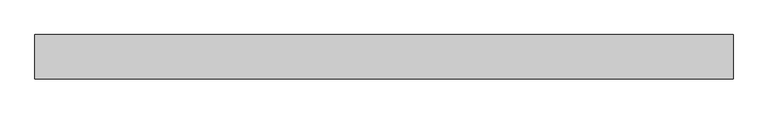
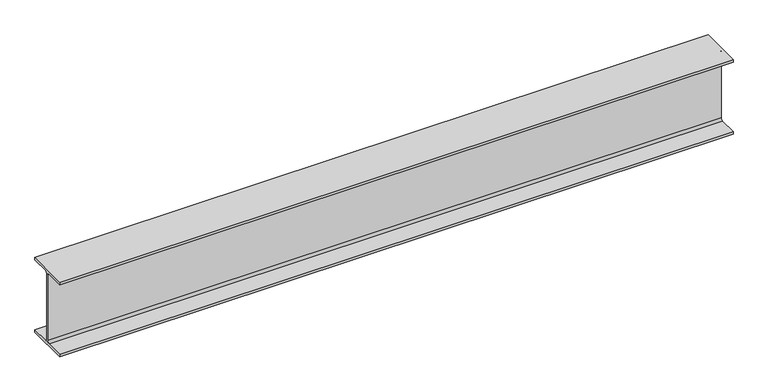
"""IFC4 building model written with IfcOpenShell, lengths in millimetres: beam geometry, Old_Steel Beam_H-KSD3502 : H_SB_ASB_H-250×125x6x9."""

import ifcopenshell
import ifcopenshell.guid

model = None  # the IFC model being written
_history = None  # IfcOwnerHistory: only IFC2X3 demands one
_inside = {}  # id of a spatial element -> (the spatial element, [elements in it])
_under = {}  # id of a project, library or spatial element -> (it, [spatial elements below it])
_declared = {}  # id of a project -> (the project, [libraries it declares])
_typed = {}  # id of a type object -> (the type object, [elements of that type])
_made_of = {}  # id of a material, layer set ... -> (it, [elements and type objects made of it])


def new_model(schema):
    """Start an empty IFC model of exactly this schema.

    Asked for "IFC4X3", IfcOpenShell would pick the latest addendum, in which some entities
    have other attributes; the version numbers below select the first issue.
    IFC2X3 requires an IfcOwnerHistory on every rooted entity: one is made here for all.
    """
    global model, _history
    if schema == "IFC4X3":
        model = ifcopenshell.file(schema_version=(4, 3, 0, 0))
    else:
        model = ifcopenshell.file(schema=schema)
    _inside.clear()
    _under.clear()
    _declared.clear()
    _typed.clear()
    _made_of.clear()
    _history = None
    if model.schema == "IFC2X3":
        org = make("IfcOrganization", Name="unknown")
        user = make(
            "IfcPersonAndOrganization",
            ThePerson=make("IfcPerson", FamilyName="unknown"),
            TheOrganization=org,
        )
        app = make(
            "IfcApplication",
            ApplicationDeveloper=org,
            Version="unknown",
            ApplicationFullName="unknown",
            ApplicationIdentifier="unknown",
        )
        _history = make(
            "IfcOwnerHistory",
            OwningUser=user,
            OwningApplication=app,
            ChangeAction="ADDED",
            CreationDate=0,
        )
    return model


def make(cls, **values):
    """One entity of the class cls with the attributes given. An attribute that is None is left unset."""
    return model.create_entity(
        cls, **{name: value for name, value in values.items() if value is not None}
    )


def rooted(cls, **values):
    """An entity with a GlobalId (a new one), such as an element, a storey or a relation."""
    return make(cls, GlobalId=ifcopenshell.guid.new(), OwnerHistory=_history, **values)


def si_unit(unit_type, name, prefix=None):
    """IfcSIUnit, for example si_unit("LENGTHUNIT", "METRE", prefix="MILLI")."""
    return make("IfcSIUnit", UnitType=unit_type, Prefix=prefix, Name=name)


def assignment(units):
    """IfcUnitAssignment: the units of a project."""
    return None if units is None else make("IfcUnitAssignment", Units=units)


def point(xyz):
    """IfcCartesianPoint."""
    return None if xyz is None else make("IfcCartesianPoint", Coordinates=xyz)


def direction(xyz):
    """IfcDirection."""
    return None if xyz is None else make("IfcDirection", DirectionRatios=xyz)


def frame(location, z_axis=None, x_axis=None):
    """IfcAxis2Placement3D, a coordinate frame: its origin and axes. An axis left out is left unset."""
    return make(
        "IfcAxis2Placement3D",
        Location=point(location),
        Axis=direction(z_axis),
        RefDirection=direction(x_axis),
    )


def frame_2d(location, x_axis=None):
    """IfcAxis2Placement2D, a coordinate frame in the plane: its origin and x axis."""
    return make(
        "IfcAxis2Placement2D", Location=point(location), RefDirection=direction(x_axis)
    )


def origin():
    """The frame at (0, 0, 0) with its axes left unset."""
    return frame((0.0, 0.0, 0.0))


def place(relative_to, where):
    """IfcLocalPlacement: puts the frame where relative to a parent placement (None: the world)."""
    return make(
        "IfcLocalPlacement", PlacementRelTo=relative_to, RelativePlacement=where
    )


def context(
    kind, dimensions, precision=None, world=None, true_north=None, identifier=None
):
    """IfcGeometricRepresentationContext, for example the 3D "Model" context."""
    return make(
        "IfcGeometricRepresentationContext",
        ContextIdentifier=identifier,
        ContextType=kind,
        CoordinateSpaceDimension=dimensions,
        Precision=precision,
        WorldCoordinateSystem=world,
        TrueNorth=true_north,
    )


def project(units=None, contexts=None):
    """IfcProject with its units and contexts."""
    return rooted(
        "IfcProject",
        Name="project",
        RepresentationContexts=contexts,
        UnitsInContext=assignment(units),
    )


def spatial(cls, under=None, at=None, **own):
    """A site, building, storey or space (cls), placed at a placement, below another one or the project."""
    s = rooted(cls, ObjectPlacement=at, **own)
    if under is not None:
        _under.setdefault(under.id(), (under, []))[1].append(s)
    return s


def polyline(points):
    """IfcPolyline through the points."""
    return make("IfcPolyline", Points=[point(p) for p in points])


def circle_curve(where, radius):
    """IfcCircle in the frame where."""
    return make("IfcCircle", Position=where, Radius=radius)


def trimmed(basis, trim1, trim2, sense, master):
    """IfcTrimmedCurve: the piece of a basis curve between two trims."""
    return make(
        "IfcTrimmedCurve",
        BasisCurve=basis,
        Trim1=trim1,
        Trim2=trim2,
        SenseAgreement=sense,
        MasterRepresentation=master,
    )


def segment(curve, same_sense, transition):
    """IfcCompositeCurveSegment."""
    return make(
        "IfcCompositeCurveSegment",
        Transition=transition,
        SameSense=same_sense,
        ParentCurve=curve,
    )


def composite_curve(segments, self_intersect=None):
    """IfcCompositeCurve: segments joined end to end."""
    return make("IfcCompositeCurve", Segments=segments, SelfIntersect=self_intersect)


def outline(outer, holes=None, kind="AREA"):
    """IfcArbitraryClosedProfileDef: a profile drawn as a closed curve; with holes, ...WithVoids."""
    if holes is None:
        return make("IfcArbitraryClosedProfileDef", ProfileType=kind, OuterCurve=outer)
    return make(
        "IfcArbitraryProfileDefWithVoids",
        ProfileType=kind,
        OuterCurve=outer,
        InnerCurves=holes,
    )


def extrude(swept, where, along, depth):
    """IfcExtrudedAreaSolid: the profile swept, set in the frame where, extruded along a direction by depth."""
    return make(
        "IfcExtrudedAreaSolid",
        SweptArea=swept,
        Position=where,
        ExtrudedDirection=direction(along),
        Depth=depth,
    )


def shape(context_of_items, identifier, shape_type, items):
    """IfcShapeRepresentation: the items that make up one representation, for example the "Body"."""
    return make(
        "IfcShapeRepresentation",
        ContextOfItems=context_of_items,
        RepresentationIdentifier=identifier,
        RepresentationType=shape_type,
        Items=items,
    )


def source(mapping_origin, context_of_items, identifier, shape_type, items):
    """IfcRepresentationMap: a shape defined once, which mapped items show again and again."""
    return make(
        "IfcRepresentationMap",
        MappingOrigin=mapping_origin,
        MappedRepresentation=shape(context_of_items, identifier, shape_type, items),
    )


def transform(
    local_origin,
    x_axis=None,
    y_axis=None,
    z_axis=None,
    scale=None,
    scale2=None,
    scale3=None,
    uniform=True,
):
    """IfcCartesianTransformationOperator3D, or its non-uniform kind. x_axis, y_axis, z_axis: its Axis1, 2, 3."""
    if uniform:
        return make(
            "IfcCartesianTransformationOperator3D",
            Axis1=direction(x_axis),
            Axis2=direction(y_axis),
            LocalOrigin=point(local_origin),
            Scale=scale,
            Axis3=direction(z_axis),
        )
    return make(
        "IfcCartesianTransformationOperator3DnonUniform",
        Axis1=direction(x_axis),
        Axis2=direction(y_axis),
        LocalOrigin=point(local_origin),
        Scale=scale,
        Axis3=direction(z_axis),
        Scale2=scale2,
        Scale3=scale3,
    )


def mapped(mapping_source, mapping_target):
    """IfcMappedItem: shows the shape of a source again, moved by a transform."""
    return make(
        "IfcMappedItem", MappingSource=mapping_source, MappingTarget=mapping_target
    )


def made_of(thing, what):
    """Note that an element or type object is made of a material, layer set ...; save() writes the relation."""
    if what is not None:
        _made_of.setdefault(what.id(), (what, []))[1].append(thing)
    return thing


def element(
    cls,
    number,
    at=None,
    inside=None,
    cuts=None,
    type_object=None,
    material=None,
    context=None,
    identifier="Body",
    shape_type=None,
    held_by="IfcProductDefinitionShape",
    body=None,
    shapes=None,
    **own,
):
    """One element of the class cls, such as IfcWall. Its Tag is "e" and its number.

    at: its placement. inside: the storey or other place that contains it. cuts: it is an
    opening in that element (IfcRelVoidsElement). A single representation is given by context,
    identifier, shape_type and body (its items); several are given by shapes. held_by: the class
    of the entity that holds the representations. save() writes the other relations.
    """
    e = rooted(cls, Tag="e%d" % number, ObjectPlacement=at, **own)
    if body is not None:
        shapes = [shape(context, identifier, shape_type, body)]
    if shapes is not None:
        e.Representation = make(held_by, Representations=shapes)
    if inside is not None:
        _inside.setdefault(inside.id(), (inside, []))[1].append(e)
    if cuts is not None:
        rooted(
            "IfcRelVoidsElement", RelatingBuildingElement=cuts, RelatedOpeningElement=e
        )
    if type_object is not None:
        _typed.setdefault(type_object.id(), (type_object, []))[1].append(e)
    return made_of(e, material)


def aggregate(whole, parts):
    """IfcRelAggregates: a whole, such as a stair, and the parts it consists of."""
    return rooted("IfcRelAggregates", RelatingObject=whole, RelatedObjects=parts)


def save(model, path):
    """Write the relations noted so far, then the file.

    IfcRelAggregates (storeys below a building ...), IfcRelContainedInSpatialStructure (elements
    in a storey), IfcRelDefinesByType, IfcRelAssociatesMaterial and IfcRelDeclares: one each for
    every whole, place, type object, material and project.
    """
    for whole, parts in _under.values():
        aggregate(whole, parts)
    for where, things in _inside.values():
        rooted(
            "IfcRelContainedInSpatialStructure",
            RelatedElements=things,
            RelatingStructure=where,
        )
    for kind, things in _typed.values():
        rooted("IfcRelDefinesByType", RelatedObjects=things, RelatingType=kind)
    for what, things in _made_of.values():
        rooted("IfcRelAssociatesMaterial", RelatedObjects=things, RelatingMaterial=what)
    for by, libraries in _declared.values():
        rooted("IfcRelDeclares", RelatingContext=by, RelatedDefinitions=libraries)
    model.write(path)


def beam_59f19b17(model_context):
    return source(origin(), model_context, "Body", "SweptSolid", [
        extrude(outline(composite_curve([segment(polyline([(82.5, -141.5), (82.5, -151.7), (-82.5, -151.7), (-82.5, -141.5), (-11.9, -141.5)]), True, "CONTINUOUS"), segment(trimmed(circle_curve(frame_2d((-11.9, -132.6)), 8.9), [point((-11.9, -141.5))], [point((-3.0, -132.6))], True, "CARTESIAN"), True, "CONTINUOUS"), segment(polyline([(-3.0, -132.6), (-3.0, 132.6)]), True, "CONTINUOUS"), segment(trimmed(circle_curve(frame_2d((-11.9, 132.6)), 8.9), [point((-3.0, 132.6))], [point((-11.9, 141.5))], True, "CARTESIAN"), True, "CONTINUOUS"), segment(polyline([(-11.9, 141.5), (-82.5, 141.5), (-82.5, 151.7), (82.5, 151.7), (82.5, 141.5), (11.9, 141.5)]), True, "CONTINUOUS"), segment(trimmed(circle_curve(frame_2d((11.9, 132.6)), 8.9), [point((11.9, 141.5))], [point((3.0, 132.6))], True, "CARTESIAN"), True, "CONTINUOUS"), segment(polyline([(3.0, 132.6), (3.0, -132.6)]), True, "CONTINUOUS"), segment(trimmed(circle_curve(frame_2d((11.9, -132.6)), 8.9), [point((3.0, -132.6))], [point((11.9, -141.5))], True, "CARTESIAN"), True, "CONTINUOUS"), segment(polyline([(11.9, -141.5), (82.5, -141.5)]), True, "CONTINUOUS")], self_intersect=False)), frame((-1249.3, 0.0, 0.0), z_axis=(1.0, 0.0, 0.0), x_axis=(0.0, 1.0, 0.0)), (0.0, 0.0, 1.0), 2586.6),
    ])


if __name__ == "__main__":
    model = new_model("IFC4")
    model_context = context("Model", 3, world=origin())
    ifc_project = project(units=[si_unit("LENGTHUNIT", "METRE", prefix="MILLI")], contexts=[model_context])
    site = spatial("IfcSite", under=ifc_project)
    building = spatial("IfcBuilding", under=site)
    placement = place(None, origin())
    beam_shape = beam_59f19b17(model_context)
    element("IfcBeam", 1, ObjectType="Old_Steel Beam_H-KSD3502 : H_SB_ASB_H-250×125x6x9", at=placement, inside=building, context=model_context, shape_type="MappedRepresentation", body=[
        mapped(beam_shape, transform((0.0, 0.0, 0.0), x_axis=(1.0, 0.0, 0.0), y_axis=(0.0, 1.0, 0.0), z_axis=(0.0, 0.0, 1.0))),
    ])
    save(model, "model.ifc")

# Revit data of these elements
# Type "Old_Steel Beam_H-KSD3502 : H_SB_ASB_H-250×125x6x9"
#   Width = 12.5 cm
#   Web Thickness = 0.6 cm
#   Web Fillet = 1.2 cm
#   Warping Constant = 42539.8 cm⁶
#   Torsional Moment of Inertia = 7.8102 cm⁴
#   Torsional Modulus = 1.0 cm³
#   Section Area = 37.66 cm²
#   Plastic Modulus weak axis = 73.1 cm³
#   Plastic Modulus strong axis = 366.0 cm³
#   Perimeter = 0.97 m²/m
#   Nominal Weight = 29.60 kgf/m
#   Moment of Inertia weak axis = 294.00 cm⁴
#   Moment of Inertia strong axis = 4050.00 cm⁴
#   Height = 25.0 cm
#   Flange Thickness = 0.9 cm
#   Elastic Modulus weak axis = 47.0 cm³
#   Elastic Modulus strong axis = 324.0 cm³
#   Centroid Vertical = 12.5 cm
#   Centroid Horizontal = 6.25 cm
#   Length [instance default] = 1.5240 m
#   Structural Material [instance default] = Steel, 45-345
#   Assembly Code = ""
# Element 1 (IfcBeam, "Old_Steel Beam_H-KSD3502 : H_SB_ASB_H-250×125x6x9")
#   Structural Material = none
# Materials
#   "Steel, 45-345": class "Metal", colour RGB 189 187 185, transparency 0, Description = "Steel 345 MPa", Cost = 0
